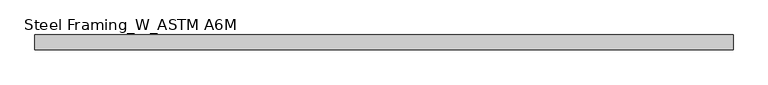
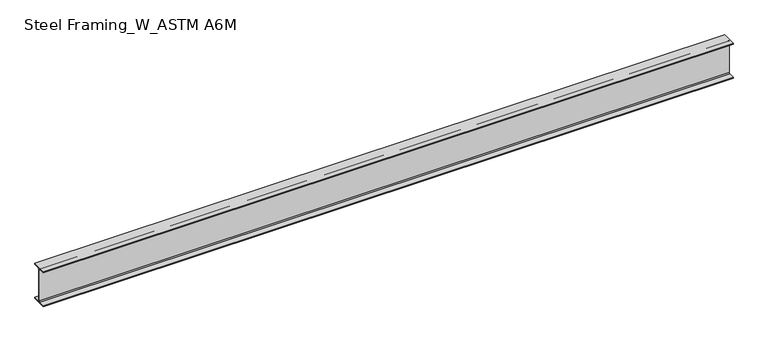
"""IFC4 building model written with IfcOpenShell, lengths in millimetres: beam geometry, Steel Framing_W_ASTM A6M : H_SB_AR_S02_W530x101_RB1."""

from ifc_helpers import new_model, si_unit, point, frame, frame_2d, origin, place, context, project, spatial, polyline, circle_curve, trimmed, segment, composite_curve, outline, extrude, source, transform, mapped, element, save


def steel_framing_w_astm_a6m_22e20aea(model_context):
    return source(origin(), model_context, "Body", "SweptSolid", [
        extrude(outline(composite_curve([segment(polyline([(105.0, -250.6), (105.0, -268.0), (-105.0, -268.0), (-105.0, -250.6), (-18.25, -250.6)]), True, "CONTINUOUS"), segment(trimmed(circle_curve(frame_2d((-18.25, -237.8)), 12.8), [point((-18.25, -250.6))], [point((-5.45, -237.8))], True, "CARTESIAN"), True, "CONTINUOUS"), segment(polyline([(-5.45, -237.8), (-5.45, 237.8)]), True, "CONTINUOUS"), segment(trimmed(circle_curve(frame_2d((-18.25, 237.8)), 12.8), [point((-5.45, 237.8))], [point((-18.25, 250.6))], True, "CARTESIAN"), True, "CONTINUOUS"), segment(polyline([(-18.25, 250.6), (-105.0, 250.6), (-105.0, 268.0), (105.0, 268.0), (105.0, 250.6), (18.25, 250.6)]), True, "CONTINUOUS"), segment(trimmed(circle_curve(frame_2d((18.25, 237.8)), 12.8), [point((18.25, 250.6))], [point((5.45, 237.8))], True, "CARTESIAN"), True, "CONTINUOUS"), segment(polyline([(5.45, 237.8), (5.45, -237.8)]), True, "CONTINUOUS"), segment(trimmed(circle_curve(frame_2d((18.25, -237.8)), 12.8), [point((5.45, -237.8))], [point((18.25, -250.6))], True, "CARTESIAN"), True, "CONTINUOUS"), segment(polyline([(18.25, -250.6), (105.0, -250.6)]), True, "CONTINUOUS")], self_intersect=False)), frame((-5000.0, 0.0, 0.0), z_axis=(1.0, 0.0, 0.0), x_axis=(0.0, 1.0, 0.0)), (0.0, 0.0, 1.0), 9987.2),
    ])


if __name__ == "__main__":
    model = new_model("IFC4")
    model_context = context("Model", 3, world=origin())
    ifc_project = project(units=[si_unit("LENGTHUNIT", "METRE", prefix="MILLI")], contexts=[model_context])
    site = spatial("IfcSite", under=ifc_project)
    building = spatial("IfcBuilding", under=site)
    placement = place(None, origin())
    steel_framing_w_astm_a6m_shape = steel_framing_w_astm_a6m_22e20aea(model_context)
    element("IfcBeam", 1, ObjectType="Steel Framing_W_ASTM A6M : H_SB_AR_S02_W530x101_RB1", at=placement, inside=building, context=model_context, shape_type="MappedRepresentation", body=[
        mapped(steel_framing_w_astm_a6m_shape, transform((0.0, 0.0, 0.0), x_axis=(1.0, 0.0, 0.0), y_axis=(0.0, 1.0, 0.0), z_axis=(0.0, 0.0, 1.0))),
    ])
    save(model, "model.ifc")

# Revit data of these elements
# Type "Steel Framing_W_ASTM A6M : H_SB_AR_S02_W530x101_RB1"
#   Type Mark = "RB1"
#   Section Name Key = "W21x68"
#   Width = 21.0 cm
#   Web Thickness = 1.09 cm
#   Web Fillet = 1.28 cm
#   Warping Constant = 1820000.0 cm⁶
#   Torsional Moment of Inertia = 102.00 cm⁴
#   Section Area = 129.0 cm²
#   Plastic Modulus weak axis = 400.0 cm³
#   Plastic Modulus strong axis = 2620.0 cm³
#   Perimeter = 1.87 m²/m
#   Nominal Weight = 101.00 kgf/m
#   Moment of Inertia weak axis = 2690.00 cm⁴
#   Moment of Inertia strong axis = 61600.00 cm⁴
#   Height = 53.6 cm
#   Flange Thickness = 1.74 cm
#   Elastic Modulus weak axis = 257.0 cm³
#   Elastic Modulus strong axis = 2290.0 cm³
#   Centroid Vertical = 26.8 cm
#   Centroid Horizontal = 10.5 cm
#   Length [instance default] = 1500 mm
#   Structural Material [instance default] = Steel, 45-345
#   Bolt Spacing = 0
#   Assembly Code = ""
# Element 1 (IfcBeam, "Steel Framing_W_ASTM A6M : H_SB_AR_S02_W530x101_RB1")
#   Materials on its faces: "Steel, 45-345"
# Materials
#   "Steel, 45-345": class "Metal", colour RGB 189 187 185, transparency 0, Description = "Steel 345 MPa", Cost = 0
